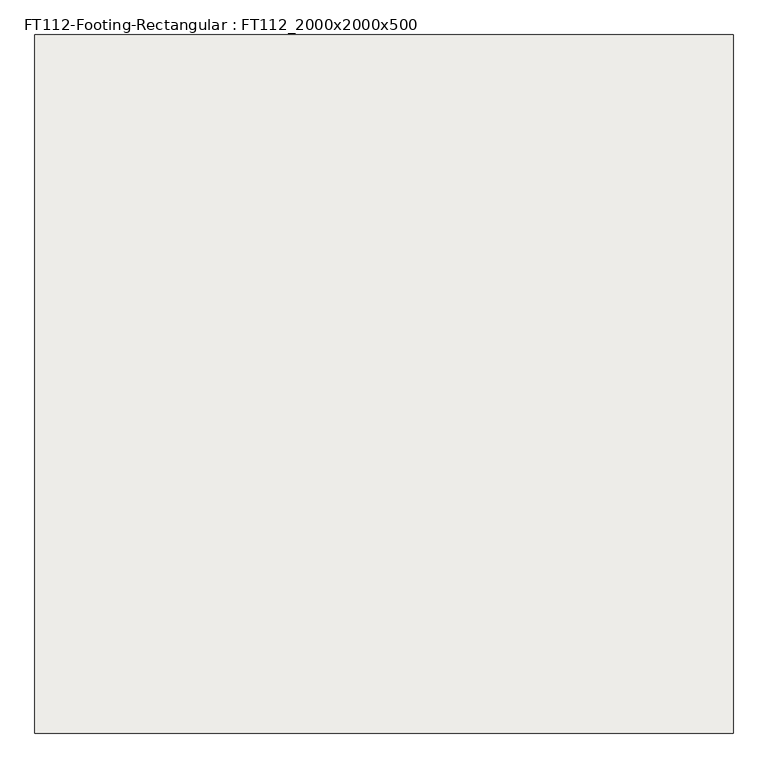
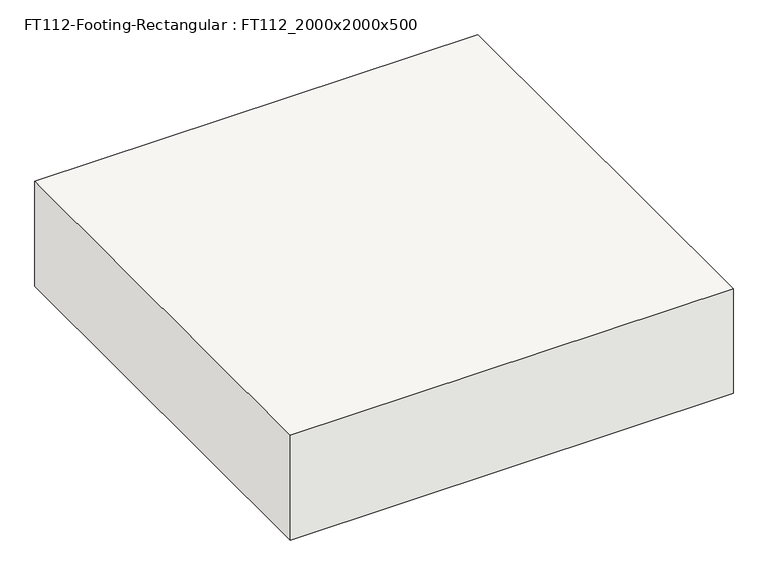
"""IFC4 building model written with IfcOpenShell, lengths in millimetres: slab geometry, FT112-Footing-Rectangular : FT112_2000x2000x500."""

import ifcopenshell
import ifcopenshell.guid

model = None  # the IFC model being written
_history = None  # IfcOwnerHistory: only IFC2X3 demands one
_inside = {}  # id of a spatial element -> (the spatial element, [elements in it])
_under = {}  # id of a project, library or spatial element -> (it, [spatial elements below it])
_declared = {}  # id of a project -> (the project, [libraries it declares])
_typed = {}  # id of a type object -> (the type object, [elements of that type])
_made_of = {}  # id of a material, layer set ... -> (it, [elements and type objects made of it])


def new_model(schema):
    """Start an empty IFC model of exactly this schema.

    Asked for "IFC4X3", IfcOpenShell would pick the latest addendum, in which some entities
    have other attributes; the version numbers below select the first issue.
    IFC2X3 requires an IfcOwnerHistory on every rooted entity: one is made here for all.
    """
    global model, _history
    if schema == "IFC4X3":
        model = ifcopenshell.file(schema_version=(4, 3, 0, 0))
    else:
        model = ifcopenshell.file(schema=schema)
    _inside.clear()
    _under.clear()
    _declared.clear()
    _typed.clear()
    _made_of.clear()
    _history = None
    if model.schema == "IFC2X3":
        org = make("IfcOrganization", Name="unknown")
        user = make(
            "IfcPersonAndOrganization",
            ThePerson=make("IfcPerson", FamilyName="unknown"),
            TheOrganization=org,
        )
        app = make(
            "IfcApplication",
            ApplicationDeveloper=org,
            Version="unknown",
            ApplicationFullName="unknown",
            ApplicationIdentifier="unknown",
        )
        _history = make(
            "IfcOwnerHistory",
            OwningUser=user,
            OwningApplication=app,
            ChangeAction="ADDED",
            CreationDate=0,
        )
    return model


def make(cls, **values):
    """One entity of the class cls with the attributes given. An attribute that is None is left unset."""
    return model.create_entity(
        cls, **{name: value for name, value in values.items() if value is not None}
    )


def rooted(cls, **values):
    """An entity with a GlobalId (a new one), such as an element, a storey or a relation."""
    return make(cls, GlobalId=ifcopenshell.guid.new(), OwnerHistory=_history, **values)


def si_unit(unit_type, name, prefix=None):
    """IfcSIUnit, for example si_unit("LENGTHUNIT", "METRE", prefix="MILLI")."""
    return make("IfcSIUnit", UnitType=unit_type, Prefix=prefix, Name=name)


def assignment(units):
    """IfcUnitAssignment: the units of a project."""
    return None if units is None else make("IfcUnitAssignment", Units=units)


def point(xyz):
    """IfcCartesianPoint."""
    return None if xyz is None else make("IfcCartesianPoint", Coordinates=xyz)


def direction(xyz):
    """IfcDirection."""
    return None if xyz is None else make("IfcDirection", DirectionRatios=xyz)


def frame(location, z_axis=None, x_axis=None):
    """IfcAxis2Placement3D, a coordinate frame: its origin and axes. An axis left out is left unset."""
    return make(
        "IfcAxis2Placement3D",
        Location=point(location),
        Axis=direction(z_axis),
        RefDirection=direction(x_axis),
    )


def origin():
    """The frame at (0, 0, 0) with its axes left unset."""
    return frame((0.0, 0.0, 0.0))


def place(relative_to, where):
    """IfcLocalPlacement: puts the frame where relative to a parent placement (None: the world)."""
    return make(
        "IfcLocalPlacement", PlacementRelTo=relative_to, RelativePlacement=where
    )


def context(
    kind, dimensions, precision=None, world=None, true_north=None, identifier=None
):
    """IfcGeometricRepresentationContext, for example the 3D "Model" context."""
    return make(
        "IfcGeometricRepresentationContext",
        ContextIdentifier=identifier,
        ContextType=kind,
        CoordinateSpaceDimension=dimensions,
        Precision=precision,
        WorldCoordinateSystem=world,
        TrueNorth=true_north,
    )


def project(units=None, contexts=None):
    """IfcProject with its units and contexts."""
    return rooted(
        "IfcProject",
        Name="project",
        RepresentationContexts=contexts,
        UnitsInContext=assignment(units),
    )


def spatial(cls, under=None, at=None, **own):
    """A site, building, storey or space (cls), placed at a placement, below another one or the project."""
    s = rooted(cls, ObjectPlacement=at, **own)
    if under is not None:
        _under.setdefault(under.id(), (under, []))[1].append(s)
    return s


def polyline(points):
    """IfcPolyline through the points."""
    return make("IfcPolyline", Points=[point(p) for p in points])


def outline(outer, holes=None, kind="AREA"):
    """IfcArbitraryClosedProfileDef: a profile drawn as a closed curve; with holes, ...WithVoids."""
    if holes is None:
        return make("IfcArbitraryClosedProfileDef", ProfileType=kind, OuterCurve=outer)
    return make(
        "IfcArbitraryProfileDefWithVoids",
        ProfileType=kind,
        OuterCurve=outer,
        InnerCurves=holes,
    )


def extrude(swept, where, along, depth):
    """IfcExtrudedAreaSolid: the profile swept, set in the frame where, extruded along a direction by depth."""
    return make(
        "IfcExtrudedAreaSolid",
        SweptArea=swept,
        Position=where,
        ExtrudedDirection=direction(along),
        Depth=depth,
    )


def shape(context_of_items, identifier, shape_type, items):
    """IfcShapeRepresentation: the items that make up one representation, for example the "Body"."""
    return make(
        "IfcShapeRepresentation",
        ContextOfItems=context_of_items,
        RepresentationIdentifier=identifier,
        RepresentationType=shape_type,
        Items=items,
    )


def source(mapping_origin, context_of_items, identifier, shape_type, items):
    """IfcRepresentationMap: a shape defined once, which mapped items show again and again."""
    return make(
        "IfcRepresentationMap",
        MappingOrigin=mapping_origin,
        MappedRepresentation=shape(context_of_items, identifier, shape_type, items),
    )


def transform(
    local_origin,
    x_axis=None,
    y_axis=None,
    z_axis=None,
    scale=None,
    scale2=None,
    scale3=None,
    uniform=True,
):
    """IfcCartesianTransformationOperator3D, or its non-uniform kind. x_axis, y_axis, z_axis: its Axis1, 2, 3."""
    if uniform:
        return make(
            "IfcCartesianTransformationOperator3D",
            Axis1=direction(x_axis),
            Axis2=direction(y_axis),
            LocalOrigin=point(local_origin),
            Scale=scale,
            Axis3=direction(z_axis),
        )
    return make(
        "IfcCartesianTransformationOperator3DnonUniform",
        Axis1=direction(x_axis),
        Axis2=direction(y_axis),
        LocalOrigin=point(local_origin),
        Scale=scale,
        Axis3=direction(z_axis),
        Scale2=scale2,
        Scale3=scale3,
    )


def mapped(mapping_source, mapping_target):
    """IfcMappedItem: shows the shape of a source again, moved by a transform."""
    return make(
        "IfcMappedItem", MappingSource=mapping_source, MappingTarget=mapping_target
    )


def made_of(thing, what):
    """Note that an element or type object is made of a material, layer set ...; save() writes the relation."""
    if what is not None:
        _made_of.setdefault(what.id(), (what, []))[1].append(thing)
    return thing


def element(
    cls,
    number,
    at=None,
    inside=None,
    cuts=None,
    type_object=None,
    material=None,
    context=None,
    identifier="Body",
    shape_type=None,
    held_by="IfcProductDefinitionShape",
    body=None,
    shapes=None,
    **own,
):
    """One element of the class cls, such as IfcWall. Its Tag is "e" and its number.

    at: its placement. inside: the storey or other place that contains it. cuts: it is an
    opening in that element (IfcRelVoidsElement). A single representation is given by context,
    identifier, shape_type and body (its items); several are given by shapes. held_by: the class
    of the entity that holds the representations. save() writes the other relations.
    """
    e = rooted(cls, Tag="e%d" % number, ObjectPlacement=at, **own)
    if body is not None:
        shapes = [shape(context, identifier, shape_type, body)]
    if shapes is not None:
        e.Representation = make(held_by, Representations=shapes)
    if inside is not None:
        _inside.setdefault(inside.id(), (inside, []))[1].append(e)
    if cuts is not None:
        rooted(
            "IfcRelVoidsElement", RelatingBuildingElement=cuts, RelatedOpeningElement=e
        )
    if type_object is not None:
        _typed.setdefault(type_object.id(), (type_object, []))[1].append(e)
    return made_of(e, material)


def aggregate(whole, parts):
    """IfcRelAggregates: a whole, such as a stair, and the parts it consists of."""
    return rooted("IfcRelAggregates", RelatingObject=whole, RelatedObjects=parts)


def save(model, path):
    """Write the relations noted so far, then the file.

    IfcRelAggregates (storeys below a building ...), IfcRelContainedInSpatialStructure (elements
    in a storey), IfcRelDefinesByType, IfcRelAssociatesMaterial and IfcRelDeclares: one each for
    every whole, place, type object, material and project.
    """
    for whole, parts in _under.values():
        aggregate(whole, parts)
    for where, things in _inside.values():
        rooted(
            "IfcRelContainedInSpatialStructure",
            RelatedElements=things,
            RelatingStructure=where,
        )
    for kind, things in _typed.values():
        rooted("IfcRelDefinesByType", RelatedObjects=things, RelatingType=kind)
    for what, things in _made_of.values():
        rooted("IfcRelAssociatesMaterial", RelatedObjects=things, RelatingMaterial=what)
    for by, libraries in _declared.values():
        rooted("IfcRelDeclares", RelatingContext=by, RelatedDefinitions=libraries)
    model.write(path)


def ft112_footing_rectangular_ft112_2000x2000x500_8ee35437(model_context):
    return source(origin(), model_context, "Body", "SweptSolid", [
        extrude(outline(polyline([(1000.0, 1000.0), (1000.0, -1000.0), (-1000.0, -1000.0), (-1000.0, 1000.0), (1000.0, 1000.0)])), frame((0.0, 0.0, -500.0), z_axis=(0.0, 0.0, 1.0), x_axis=(1.0, 0.0, 0.0)), (0.0, 0.0, 1.0), 500.0),
    ])


if __name__ == "__main__":
    model = new_model("IFC4")
    model_context = context("Model", 3, world=origin())
    ifc_project = project(units=[si_unit("LENGTHUNIT", "METRE", prefix="MILLI")], contexts=[model_context])
    site = spatial("IfcSite", under=ifc_project)
    building = spatial("IfcBuilding", under=site)
    placement = place(None, origin())
    ft112_footing_rectangular_ft112_2000x2000x500_shape = ft112_footing_rectangular_ft112_2000x2000x500_8ee35437(model_context)
    element("IfcSlab", 1, ObjectType="FT112-Footing-Rectangular : FT112_2000x2000x500", at=placement, inside=building, context=model_context, shape_type="MappedRepresentation", body=[
        mapped(ft112_footing_rectangular_ft112_2000x2000x500_shape, transform((0.0, 0.0, 0.0), x_axis=(1.0, 0.0, 0.0), y_axis=(0.0, 1.0, 0.0), z_axis=(0.0, 0.0, 1.0))),
    ])
    save(model, "model.ifc")

# Revit data of these elements
# Type "FT112-Footing-Rectangular : FT112_2000x2000x500"
#   Description = "UG Shallow Foundation"
#   Description = "UG Shallow Foundation"
#   Width = 2000 mm
#   Length = 2000 mm
#   Foundation Thickness = 500 mm
#   hec_material3 [instance default] = none
#   hec_material2 [instance default] = A03AE056-00001_Bitumen/Bituminous/Asphalt Coating
#   hec_material1 [instance default] = A03AC035-00001_Form Work (3 times in use)_Flat
#   Structural Material [instance default] = A03AC032-00007_Structural Concrete_Type1_25MPa-30Mpa
#   Assembly Code = ""
# Element 1 (IfcSlab, "FT112-Footing-Rectangular : FT112_2000x2000x500")
#   Structural Material = 콘크리트 - 현장타설 콘크리트
#   Materials on its faces: "콘크리트 - 현장타설 콘크리트"
# Materials
#   "A03AE056-00001_Bitumen/Bituminous/Asphalt Coating": class "Generic", colour RGB 17 17 17, transparency 0, Description = "Damp-proofing", W00) Work Master Code = "A03AE056-00001", W01) Work Master_Lv1 = "Concrete Work", W02) Work Master_Lv2 = "Concrete Protective Coating (U/G)", W03) Work Master_Spec.1 = "Bitumen/Bituminous/Asphalt Coating", Cost = 0
#   "A03AC035-00001_Form Work (3 times in use)_Flat": class "Wood", colour RGB 149 120 74, transparency 0, Description = "Plywood", W00) Work Master Code = "A03AC035-00001", W01) Work Master_Lv1 = "Concrete Work", W02) Work Master_Lv2 = "Substructure Work", W03) Work Master_Spec.1 = "Form Work (3 times in use)", W04) Work Master_Spec.2 = "Flat Form", W05) Work Master_Spec.3 = "Dressed Lumber, Plywood or Steel Form(Wood Planks are not Allowed) incl. Chamfer", Cost = 0
#   "A03AC032-00007_Structural Concrete_Type1_25MPa-30Mpa": class "Concrete", colour RGB 176 176 176, transparency 0, Keynote = "09910.A1", Description = "Reinf. Conc.", W00) Work Master Code = "A03AC032-00007", W01) Work Master_Lv1 = "Concrete Work", W02) Work Master_Lv2 = "Substructure Work", W03) Work Master_Spec.1 = "Structural Concrete", W04) Work Master_Spec.2 = "Cement Type-1", W05) Work Master_Spec.3 = "25MPa < F'c (Cylinder Strength) ≤ 30MPa", Cost = 0
#   "콘크리트 - 현장타설 콘크리트": class "콘크리트", colour RGB 192 192 192, transparency 0, Cost = 0
